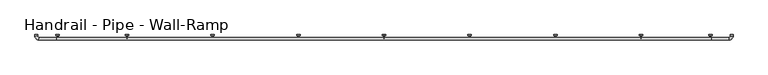
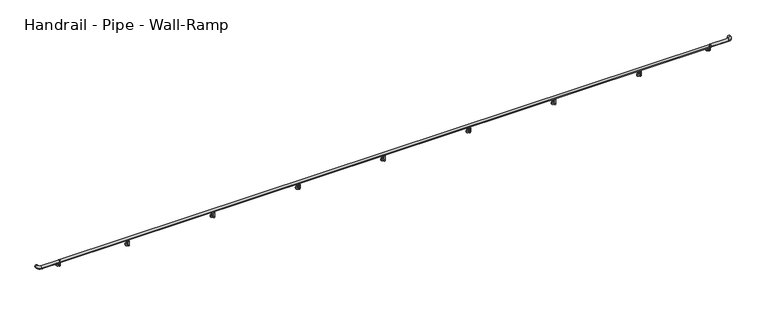
"""IFC4 building model written with IfcOpenShell, lengths in millimetres: railing geometry, Handrail - Pipe - Wall-Ramp."""

from ifc_helpers import new_model, si_unit, point, frame, frame_2d, origin, place, context, project, spatial, circle_curve, ellipse_curve, trimmed, segment, composite_curve, outline, extrude, source, transform, mapped, element, save
from ifc_brep_helpers import plane_surface, cylinder_surface, revolved_surface, advanced_brep


def handrail_pipe_wall_ramp_020da921(model_context):
    return source(origin(), model_context, "Body", "SolidModel", [
        extrude(outline(composite_curve([segment(trimmed(circle_curve(frame_2d((5007.0738685, 895.35)), 19.05), [point((4988.0238685, 895.35))], [point((5026.1238685, 895.35))], False, "CARTESIAN"), True, "CONTINUOUS"), segment(trimmed(circle_curve(frame_2d((5007.0738685, 895.35)), 19.05), [point((5026.1238685, 895.35))], [point((4988.0238685, 895.35))], False, "CARTESIAN"), True, "CONTINUOUS")], self_intersect=False)), frame((-2498.891568, 0.0, 0.0), z_axis=(1.0, 0.0, 0.0), x_axis=(0.0, 1.0, 0.0)), (0.0, 0.0, 1.0), 9315.45),
        advanced_brep(
        [(-1492.416568, 5007.0738685, 857.25), (-1505.116568, 5007.0738685, 857.25), (-1492.416568, 5007.0738685, 800.1), (-1505.116568, 5007.0738685, 800.1), (-1505.116568, 5026.1238685, 781.05), (-1492.416568, 5026.1238685, 781.05), (-1492.416568, 5054.6988685, 781.05), (-1505.116568, 5054.6988685, 781.05)],
        [
            (0, 1, circle_curve(frame((-1498.766568, 5007.0738685, 857.25), z_axis=(0.0, 0.0, 1.0), x_axis=(-1.0, 0.0, 0.0)), 6.35)),
            (1, 0, circle_curve(frame((-1498.766568, 5007.0738685, 857.25), z_axis=(0.0, 0.0, 1.0), x_axis=(-1.0, 0.0, 0.0)), 6.35)),
            (0, 2),
            (2, 3, circle_curve(frame((-1498.766568, 5007.0738685, 800.1), z_axis=(0.0, 0.0, 1.0), x_axis=(-1.0, 0.0, 0.0)), 6.35)),
            (3, 1),
            (3, 2, circle_curve(frame((-1498.766568, 5007.0738685, 800.1), z_axis=(0.0, 0.0, 1.0), x_axis=(-1.0, 0.0, 0.0)), 6.35)),
            (4, 3, circle_curve(frame((-1505.116568, 5026.1238685, 800.1), z_axis=(-1.0, 0.0, 0.0), x_axis=(0.0, -1.0, 0.0)), 19.05)),
            (2, 5, circle_curve(frame((-1492.416568, 5026.1238685, 800.1), z_axis=(1.0, 0.0, 0.0), x_axis=(0.0, -1.0, 0.0)), 19.05)),
            (5, 4, circle_curve(frame((-1498.766568, 5026.1238685, 781.05), z_axis=(0.0, -1.0, 0.0), x_axis=(-1.0, 0.0, 0.0)), 6.35)),
            (4, 5, circle_curve(frame((-1498.766568, 5026.1238685, 781.05), z_axis=(0.0, -1.0, 0.0), x_axis=(-1.0, 0.0, 0.0)), 6.35)),
            (6, 7, circle_curve(frame((-1498.766568, 5054.6988685, 781.05), z_axis=(0.0, 1.0, 0.0), x_axis=(-1.0, 0.0, 0.0)), 6.35)),
            (7, 6, circle_curve(frame((-1498.766568, 5054.6988685, 781.05), z_axis=(0.0, 1.0, 0.0), x_axis=(-1.0, 0.0, 0.0)), 6.35)),
            (5, 6),
            (7, 4),
        ],
        [
            plane_surface(frame((-1505.116568, 5007.0738685, 857.25), z_axis=(0.0, 0.0, 1.0), x_axis=(0.0, 1.0, 0.0))),
            cylinder_surface(frame((-1498.766568, 5007.0738685, 857.25), z_axis=(0.0, 0.0, 1.0), x_axis=(-1.0, 0.0, 0.0)), 6.35),
            revolved_surface(trimmed(ellipse_curve(frame((-1498.766568, 5007.0738685, 800.1), z_axis=(0.0, 0.0, 1.0), x_axis=(-1.0, 0.0, 0.0)), 6.35, 6.35), [point((-1492.416568, 5007.0738685, 800.1))], [point((-1505.116568, 5007.0738685, 800.1))], True, "CARTESIAN"), (-1498.766568, 5026.1238685, 800.1), (1.0, 0.0, 0.0)),
            revolved_surface(trimmed(ellipse_curve(frame((-1498.766568, 5007.0738685, 800.1), z_axis=(0.0, 0.0, 1.0), x_axis=(-1.0, 0.0, 0.0)), 6.35, 6.35), [point((-1505.116568, 5007.0738685, 800.1))], [point((-1492.416568, 5007.0738685, 800.1))], True, "CARTESIAN"), (-1498.766568, 5026.1238685, 800.1), (1.0, 0.0, 0.0)),
            plane_surface(frame((-1498.766568, 5054.6988685, 774.7), z_axis=(0.0, 1.0, 0.0), x_axis=(-1.0, 0.0, 0.0))),
            cylinder_surface(frame((-1498.766568, 5026.1238685, 781.05), z_axis=(0.0, -1.0, 0.0), x_axis=(-1.0, 0.0, 0.0)), 6.35),
        ],
        [
            (0, [[1, 2]]),
            (1, [[-1, 3, 4, 5]]),
            (1, [[-2, -5, 6, -3]]),
            (2, [[7, -4, 8, 9]]),
            (3, [[-8, -6, -7, 10]]),
            (4, [[11, 12]]),
            (5, [[-9, 13, -12, 14]]),
            (5, [[-10, -14, -11, -13]]),
        ],
    ),
        extrude(outline(composite_curve([segment(trimmed(circle_curve(frame_2d((781.05, -1498.766568)), 25.4), [point((781.05, -1524.166568))], [point((781.05, -1473.366568))], False, "CARTESIAN"), True, "CONTINUOUS"), segment(trimmed(circle_curve(frame_2d((781.05, -1498.766568)), 25.4), [point((781.05, -1473.366568))], [point((781.05, -1524.166568))], False, "CARTESIAN"), True, "CONTINUOUS")], self_intersect=False)), frame((0.0, 5054.6988685, 0.0), z_axis=(0.0, 1.0, 0.0), x_axis=(0.0, 0.0, 1.0)), (0.0, 0.0, 1.0), 9.525),
        advanced_brep(
        [(-273.216568, 5007.0738685, 857.25), (-285.916568, 5007.0738685, 857.25), (-273.216568, 5007.0738685, 800.1), (-285.916568, 5007.0738685, 800.1), (-285.916568, 5026.1238685, 781.05), (-273.216568, 5026.1238685, 781.05), (-273.216568, 5054.6988685, 781.05), (-285.916568, 5054.6988685, 781.05)],
        [
            (0, 1, circle_curve(frame((-279.566568, 5007.0738685, 857.25), z_axis=(0.0, 0.0, 1.0), x_axis=(-1.0, 0.0, 0.0)), 6.35)),
            (1, 0, circle_curve(frame((-279.566568, 5007.0738685, 857.25), z_axis=(0.0, 0.0, 1.0), x_axis=(-1.0, 0.0, 0.0)), 6.35)),
            (0, 2),
            (2, 3, circle_curve(frame((-279.566568, 5007.0738685, 800.1), z_axis=(0.0, 0.0, 1.0), x_axis=(-1.0, 0.0, 0.0)), 6.35)),
            (3, 1),
            (3, 2, circle_curve(frame((-279.566568, 5007.0738685, 800.1), z_axis=(0.0, 0.0, 1.0), x_axis=(-1.0, 0.0, 0.0)), 6.35)),
            (4, 3, circle_curve(frame((-285.916568, 5026.1238685, 800.1), z_axis=(-1.0, 0.0, 0.0), x_axis=(0.0, -1.0, 0.0)), 19.05)),
            (2, 5, circle_curve(frame((-273.216568, 5026.1238685, 800.1), z_axis=(1.0, 0.0, 0.0), x_axis=(0.0, -1.0, 0.0)), 19.05)),
            (5, 4, circle_curve(frame((-279.566568, 5026.1238685, 781.05), z_axis=(0.0, -1.0, 0.0), x_axis=(-1.0, 0.0, 0.0)), 6.35)),
            (4, 5, circle_curve(frame((-279.566568, 5026.1238685, 781.05), z_axis=(0.0, -1.0, 0.0), x_axis=(-1.0, 0.0, 0.0)), 6.35)),
            (6, 7, circle_curve(frame((-279.566568, 5054.6988685, 781.05), z_axis=(0.0, 1.0, 0.0), x_axis=(-1.0, 0.0, 0.0)), 6.35)),
            (7, 6, circle_curve(frame((-279.566568, 5054.6988685, 781.05), z_axis=(0.0, 1.0, 0.0), x_axis=(-1.0, 0.0, 0.0)), 6.35)),
            (5, 6),
            (7, 4),
        ],
        [
            plane_surface(frame((-285.916568, 5007.0738685, 857.25), z_axis=(0.0, 0.0, 1.0), x_axis=(0.0, 1.0, 0.0))),
            cylinder_surface(frame((-279.566568, 5007.0738685, 857.25), z_axis=(0.0, 0.0, 1.0), x_axis=(-1.0, 0.0, 0.0)), 6.35),
            revolved_surface(trimmed(ellipse_curve(frame((-279.566568, 5007.0738685, 800.1), z_axis=(0.0, 0.0, 1.0), x_axis=(-1.0, 0.0, 0.0)), 6.35, 6.35), [point((-273.216568, 5007.0738685, 800.1))], [point((-285.916568, 5007.0738685, 800.1))], True, "CARTESIAN"), (-279.566568, 5026.1238685, 800.1), (1.0, 0.0, 0.0)),
            revolved_surface(trimmed(ellipse_curve(frame((-279.566568, 5007.0738685, 800.1), z_axis=(0.0, 0.0, 1.0), x_axis=(-1.0, 0.0, 0.0)), 6.35, 6.35), [point((-285.916568, 5007.0738685, 800.1))], [point((-273.216568, 5007.0738685, 800.1))], True, "CARTESIAN"), (-279.566568, 5026.1238685, 800.1), (1.0, 0.0, 0.0)),
            plane_surface(frame((-279.566568, 5054.6988685, 774.7), z_axis=(0.0, 1.0, 0.0), x_axis=(-1.0, 0.0, 0.0))),
            cylinder_surface(frame((-279.566568, 5026.1238685, 781.05), z_axis=(0.0, -1.0, 0.0), x_axis=(-1.0, 0.0, 0.0)), 6.35),
        ],
        [
            (0, [[1, 2]]),
            (1, [[-1, 3, 4, 5]]),
            (1, [[-2, -5, 6, -3]]),
            (2, [[7, -4, 8, 9]]),
            (3, [[-8, -6, -7, 10]]),
            (4, [[11, 12]]),
            (5, [[-9, 13, -12, 14]]),
            (5, [[-10, -14, -11, -13]]),
        ],
    ),
        extrude(outline(composite_curve([segment(trimmed(circle_curve(frame_2d((781.05, -279.566568)), 25.4), [point((781.05, -304.966568))], [point((781.05, -254.166568))], False, "CARTESIAN"), True, "CONTINUOUS"), segment(trimmed(circle_curve(frame_2d((781.05, -279.566568)), 25.4), [point((781.05, -254.166568))], [point((781.05, -304.966568))], False, "CARTESIAN"), True, "CONTINUOUS")], self_intersect=False)), frame((0.0, 5054.6988685, 0.0), z_axis=(0.0, 1.0, 0.0), x_axis=(0.0, 0.0, 1.0)), (0.0, 0.0, 1.0), 9.525),
        advanced_brep(
        [(945.983432, 5007.0738685, 857.25), (933.283432, 5007.0738685, 857.25), (945.983432, 5007.0738685, 800.1), (933.283432, 5007.0738685, 800.1), (933.283432, 5026.1238685, 781.05), (945.983432, 5026.1238685, 781.05), (945.983432, 5054.6988685, 781.05), (933.283432, 5054.6988685, 781.05)],
        [
            (0, 1, circle_curve(frame((939.633432, 5007.0738685, 857.25), z_axis=(0.0, 0.0, 1.0), x_axis=(-1.0, 0.0, 0.0)), 6.35)),
            (1, 0, circle_curve(frame((939.633432, 5007.0738685, 857.25), z_axis=(0.0, 0.0, 1.0), x_axis=(-1.0, 0.0, 0.0)), 6.35)),
            (0, 2),
            (2, 3, circle_curve(frame((939.633432, 5007.0738685, 800.1), z_axis=(0.0, 0.0, 1.0), x_axis=(-1.0, 0.0, 0.0)), 6.35)),
            (3, 1),
            (3, 2, circle_curve(frame((939.633432, 5007.0738685, 800.1), z_axis=(0.0, 0.0, 1.0), x_axis=(-1.0, 0.0, 0.0)), 6.35)),
            (4, 3, circle_curve(frame((933.283432, 5026.1238685, 800.1), z_axis=(-1.0, 0.0, 0.0), x_axis=(0.0, -1.0, 0.0)), 19.05)),
            (2, 5, circle_curve(frame((945.983432, 5026.1238685, 800.1), z_axis=(1.0, 0.0, 0.0), x_axis=(0.0, -1.0, 0.0)), 19.05)),
            (5, 4, circle_curve(frame((939.633432, 5026.1238685, 781.05), z_axis=(0.0, -1.0, 0.0), x_axis=(-1.0, 0.0, 0.0)), 6.35)),
            (4, 5, circle_curve(frame((939.633432, 5026.1238685, 781.05), z_axis=(0.0, -1.0, 0.0), x_axis=(-1.0, 0.0, 0.0)), 6.35)),
            (6, 7, circle_curve(frame((939.633432, 5054.6988685, 781.05), z_axis=(0.0, 1.0, 0.0), x_axis=(-1.0, 0.0, 0.0)), 6.35)),
            (7, 6, circle_curve(frame((939.633432, 5054.6988685, 781.05), z_axis=(0.0, 1.0, 0.0), x_axis=(-1.0, 0.0, 0.0)), 6.35)),
            (5, 6),
            (7, 4),
        ],
        [
            plane_surface(frame((933.283432, 5007.0738685, 857.25), z_axis=(0.0, 0.0, 1.0), x_axis=(0.0, 1.0, 0.0))),
            cylinder_surface(frame((939.633432, 5007.0738685, 857.25), z_axis=(0.0, 0.0, 1.0), x_axis=(-1.0, 0.0, 0.0)), 6.35),
            revolved_surface(trimmed(ellipse_curve(frame((939.633432, 5007.0738685, 800.1), z_axis=(0.0, 0.0, 1.0), x_axis=(-1.0, 0.0, 0.0)), 6.35, 6.35), [point((945.983432, 5007.0738685, 800.1))], [point((933.283432, 5007.0738685, 800.1))], True, "CARTESIAN"), (939.633432, 5026.1238685, 800.1), (1.0, 0.0, 0.0)),
            revolved_surface(trimmed(ellipse_curve(frame((939.633432, 5007.0738685, 800.1), z_axis=(0.0, 0.0, 1.0), x_axis=(-1.0, 0.0, 0.0)), 6.35, 6.35), [point((933.283432, 5007.0738685, 800.1))], [point((945.983432, 5007.0738685, 800.1))], True, "CARTESIAN"), (939.633432, 5026.1238685, 800.1), (1.0, 0.0, 0.0)),
            plane_surface(frame((939.633432, 5054.6988685, 774.7), z_axis=(0.0, 1.0, 0.0), x_axis=(-1.0, 0.0, 0.0))),
            cylinder_surface(frame((939.633432, 5026.1238685, 781.05), z_axis=(0.0, -1.0, 0.0), x_axis=(-1.0, 0.0, 0.0)), 6.35),
        ],
        [
            (0, [[1, 2]]),
            (1, [[-1, 3, 4, 5]]),
            (1, [[-2, -5, 6, -3]]),
            (2, [[7, -4, 8, 9]]),
            (3, [[-8, -6, -7, 10]]),
            (4, [[11, 12]]),
            (5, [[-9, 13, -12, 14]]),
            (5, [[-10, -14, -11, -13]]),
        ],
    ),
        extrude(outline(composite_curve([segment(trimmed(circle_curve(frame_2d((781.05, 939.633432)), 25.4), [point((781.05, 914.233432))], [point((781.05, 965.033432))], False, "CARTESIAN"), True, "CONTINUOUS"), segment(trimmed(circle_curve(frame_2d((781.05, 939.633432)), 25.4), [point((781.05, 965.033432))], [point((781.05, 914.233432))], False, "CARTESIAN"), True, "CONTINUOUS")], self_intersect=False)), frame((0.0, 5054.6988685, 0.0), z_axis=(0.0, 1.0, 0.0), x_axis=(0.0, 0.0, 1.0)), (0.0, 0.0, 1.0), 9.525),
        advanced_brep(
        [(2165.183432, 5007.0738685, 857.25), (2152.483432, 5007.0738685, 857.25), (2165.183432, 5007.0738685, 800.1), (2152.483432, 5007.0738685, 800.1), (2152.483432, 5026.1238685, 781.05), (2165.183432, 5026.1238685, 781.05), (2165.183432, 5054.6988685, 781.05), (2152.483432, 5054.6988685, 781.05)],
        [
            (0, 1, circle_curve(frame((2158.833432, 5007.0738685, 857.25), z_axis=(0.0, 0.0, 1.0), x_axis=(-1.0, 0.0, 0.0)), 6.35)),
            (1, 0, circle_curve(frame((2158.833432, 5007.0738685, 857.25), z_axis=(0.0, 0.0, 1.0), x_axis=(-1.0, 0.0, 0.0)), 6.35)),
            (0, 2),
            (2, 3, circle_curve(frame((2158.833432, 5007.0738685, 800.1), z_axis=(0.0, 0.0, 1.0), x_axis=(-1.0, 0.0, 0.0)), 6.35)),
            (3, 1),
            (3, 2, circle_curve(frame((2158.833432, 5007.0738685, 800.1), z_axis=(0.0, 0.0, 1.0), x_axis=(-1.0, 0.0, 0.0)), 6.35)),
            (4, 3, circle_curve(frame((2152.483432, 5026.1238685, 800.1), z_axis=(-1.0, 0.0, 0.0), x_axis=(0.0, -1.0, 0.0)), 19.05)),
            (2, 5, circle_curve(frame((2165.183432, 5026.1238685, 800.1), z_axis=(1.0, 0.0, 0.0), x_axis=(0.0, -1.0, 0.0)), 19.05)),
            (5, 4, circle_curve(frame((2158.833432, 5026.1238685, 781.05), z_axis=(0.0, -1.0, 0.0), x_axis=(-1.0, 0.0, 0.0)), 6.35)),
            (4, 5, circle_curve(frame((2158.833432, 5026.1238685, 781.05), z_axis=(0.0, -1.0, 0.0), x_axis=(-1.0, 0.0, 0.0)), 6.35)),
            (6, 7, circle_curve(frame((2158.833432, 5054.6988685, 781.05), z_axis=(0.0, 1.0, 0.0), x_axis=(-1.0, 0.0, 0.0)), 6.35)),
            (7, 6, circle_curve(frame((2158.833432, 5054.6988685, 781.05), z_axis=(0.0, 1.0, 0.0), x_axis=(-1.0, 0.0, 0.0)), 6.35)),
            (5, 6),
            (7, 4),
        ],
        [
            plane_surface(frame((2152.483432, 5007.0738685, 857.25), z_axis=(0.0, 0.0, 1.0), x_axis=(0.0, 1.0, 0.0))),
            cylinder_surface(frame((2158.833432, 5007.0738685, 857.25), z_axis=(0.0, 0.0, 1.0), x_axis=(-1.0, 0.0, 0.0)), 6.35),
            revolved_surface(trimmed(ellipse_curve(frame((2158.833432, 5007.0738685, 800.1), z_axis=(0.0, 0.0, 1.0), x_axis=(-1.0, 0.0, 0.0)), 6.35, 6.35), [point((2165.183432, 5007.0738685, 800.1))], [point((2152.483432, 5007.0738685, 800.1))], True, "CARTESIAN"), (2158.833432, 5026.1238685, 800.1), (1.0, 0.0, 0.0)),
            revolved_surface(trimmed(ellipse_curve(frame((2158.833432, 5007.0738685, 800.1), z_axis=(0.0, 0.0, 1.0), x_axis=(-1.0, 0.0, 0.0)), 6.35, 6.35), [point((2152.483432, 5007.0738685, 800.1))], [point((2165.183432, 5007.0738685, 800.1))], True, "CARTESIAN"), (2158.833432, 5026.1238685, 800.1), (1.0, 0.0, 0.0)),
            plane_surface(frame((2158.833432, 5054.6988685, 774.7), z_axis=(0.0, 1.0, 0.0), x_axis=(-1.0, 0.0, 0.0))),
            cylinder_surface(frame((2158.833432, 5026.1238685, 781.05), z_axis=(0.0, -1.0, 0.0), x_axis=(-1.0, 0.0, 0.0)), 6.35),
        ],
        [
            (0, [[1, 2]]),
            (1, [[-1, 3, 4, 5]]),
            (1, [[-2, -5, 6, -3]]),
            (2, [[7, -4, 8, 9]]),
            (3, [[-8, -6, -7, 10]]),
            (4, [[11, 12]]),
            (5, [[-9, 13, -12, 14]]),
            (5, [[-10, -14, -11, -13]]),
        ],
    ),
        extrude(outline(composite_curve([segment(trimmed(circle_curve(frame_2d((781.05, 2158.833432)), 25.4), [point((781.05, 2133.433432))], [point((781.05, 2184.233432))], False, "CARTESIAN"), True, "CONTINUOUS"), segment(trimmed(circle_curve(frame_2d((781.05, 2158.833432)), 25.4), [point((781.05, 2184.233432))], [point((781.05, 2133.433432))], False, "CARTESIAN"), True, "CONTINUOUS")], self_intersect=False)), frame((0.0, 5054.6988685, 0.0), z_axis=(0.0, 1.0, 0.0), x_axis=(0.0, 0.0, 1.0)), (0.0, 0.0, 1.0), 9.525),
        advanced_brep(
        [(3384.383432, 5007.0738685, 857.25), (3371.683432, 5007.0738685, 857.25), (3384.383432, 5007.0738685, 800.1), (3371.683432, 5007.0738685, 800.1), (3371.683432, 5026.1238685, 781.05), (3384.383432, 5026.1238685, 781.05), (3384.383432, 5054.6988685, 781.05), (3371.683432, 5054.6988685, 781.05)],
        [
            (0, 1, circle_curve(frame((3378.033432, 5007.0738685, 857.25), z_axis=(0.0, 0.0, 1.0), x_axis=(-1.0, 0.0, 0.0)), 6.35)),
            (1, 0, circle_curve(frame((3378.033432, 5007.0738685, 857.25), z_axis=(0.0, 0.0, 1.0), x_axis=(-1.0, 0.0, 0.0)), 6.35)),
            (0, 2),
            (2, 3, circle_curve(frame((3378.033432, 5007.0738685, 800.1), z_axis=(0.0, 0.0, 1.0), x_axis=(-1.0, 0.0, 0.0)), 6.35)),
            (3, 1),
            (3, 2, circle_curve(frame((3378.033432, 5007.0738685, 800.1), z_axis=(0.0, 0.0, 1.0), x_axis=(-1.0, 0.0, 0.0)), 6.35)),
            (4, 3, circle_curve(frame((3371.683432, 5026.1238685, 800.1), z_axis=(-1.0, 0.0, 0.0), x_axis=(0.0, -1.0, 0.0)), 19.05)),
            (2, 5, circle_curve(frame((3384.383432, 5026.1238685, 800.1), z_axis=(1.0, 0.0, 0.0), x_axis=(0.0, -1.0, 0.0)), 19.05)),
            (5, 4, circle_curve(frame((3378.033432, 5026.1238685, 781.05), z_axis=(0.0, -1.0, 0.0), x_axis=(-1.0, 0.0, 0.0)), 6.35)),
            (4, 5, circle_curve(frame((3378.033432, 5026.1238685, 781.05), z_axis=(0.0, -1.0, 0.0), x_axis=(-1.0, 0.0, 0.0)), 6.35)),
            (6, 7, circle_curve(frame((3378.033432, 5054.6988685, 781.05), z_axis=(0.0, 1.0, 0.0), x_axis=(-1.0, 0.0, 0.0)), 6.35)),
            (7, 6, circle_curve(frame((3378.033432, 5054.6988685, 781.05), z_axis=(0.0, 1.0, 0.0), x_axis=(-1.0, 0.0, 0.0)), 6.35)),
            (5, 6),
            (7, 4),
        ],
        [
            plane_surface(frame((3371.683432, 5007.0738685, 857.25), z_axis=(0.0, 0.0, 1.0), x_axis=(0.0, 1.0, 0.0))),
            cylinder_surface(frame((3378.033432, 5007.0738685, 857.25), z_axis=(0.0, 0.0, 1.0), x_axis=(-1.0, 0.0, 0.0)), 6.35),
            revolved_surface(trimmed(ellipse_curve(frame((3378.033432, 5007.0738685, 800.1), z_axis=(0.0, 0.0, 1.0), x_axis=(-1.0, 0.0, 0.0)), 6.35, 6.35), [point((3384.383432, 5007.0738685, 800.1))], [point((3371.683432, 5007.0738685, 800.1))], True, "CARTESIAN"), (3378.033432, 5026.1238685, 800.1), (1.0, 0.0, 0.0)),
            revolved_surface(trimmed(ellipse_curve(frame((3378.033432, 5007.0738685, 800.1), z_axis=(0.0, 0.0, 1.0), x_axis=(-1.0, 0.0, 0.0)), 6.35, 6.35), [point((3371.683432, 5007.0738685, 800.1))], [point((3384.383432, 5007.0738685, 800.1))], True, "CARTESIAN"), (3378.033432, 5026.1238685, 800.1), (1.0, 0.0, 0.0)),
            plane_surface(frame((3378.033432, 5054.6988685, 774.7), z_axis=(0.0, 1.0, 0.0), x_axis=(-1.0, 0.0, 0.0))),
            cylinder_surface(frame((3378.033432, 5026.1238685, 781.05), z_axis=(0.0, -1.0, 0.0), x_axis=(-1.0, 0.0, 0.0)), 6.35),
        ],
        [
            (0, [[1, 2]]),
            (1, [[-1, 3, 4, 5]]),
            (1, [[-2, -5, 6, -3]]),
            (2, [[7, -4, 8, 9]]),
            (3, [[-8, -6, -7, 10]]),
            (4, [[11, 12]]),
            (5, [[-9, 13, -12, 14]]),
            (5, [[-10, -14, -11, -13]]),
        ],
    ),
        extrude(outline(composite_curve([segment(trimmed(circle_curve(frame_2d((781.05, 3378.033432)), 25.4), [point((781.05, 3352.633432))], [point((781.05, 3403.433432))], False, "CARTESIAN"), True, "CONTINUOUS"), segment(trimmed(circle_curve(frame_2d((781.05, 3378.033432)), 25.4), [point((781.05, 3403.433432))], [point((781.05, 3352.633432))], False, "CARTESIAN"), True, "CONTINUOUS")], self_intersect=False)), frame((0.0, 5054.6988685, 0.0), z_axis=(0.0, 1.0, 0.0), x_axis=(0.0, 0.0, 1.0)), (0.0, 0.0, 1.0), 9.525),
        advanced_brep(
        [(4603.583432, 5007.0738685, 857.25), (4590.883432, 5007.0738685, 857.25), (4603.583432, 5007.0738685, 800.1), (4590.883432, 5007.0738685, 800.1), (4590.883432, 5026.1238685, 781.05), (4603.583432, 5026.1238685, 781.05), (4603.583432, 5054.6988685, 781.05), (4590.883432, 5054.6988685, 781.05)],
        [
            (0, 1, circle_curve(frame((4597.233432, 5007.0738685, 857.25), z_axis=(0.0, 0.0, 1.0), x_axis=(-1.0, 0.0, 0.0)), 6.35)),
            (1, 0, circle_curve(frame((4597.233432, 5007.0738685, 857.25), z_axis=(0.0, 0.0, 1.0), x_axis=(-1.0, 0.0, 0.0)), 6.35)),
            (0, 2),
            (2, 3, circle_curve(frame((4597.233432, 5007.0738685, 800.1), z_axis=(0.0, 0.0, 1.0), x_axis=(-1.0, 0.0, 0.0)), 6.35)),
            (3, 1),
            (3, 2, circle_curve(frame((4597.233432, 5007.0738685, 800.1), z_axis=(0.0, 0.0, 1.0), x_axis=(-1.0, 0.0, 0.0)), 6.35)),
            (4, 3, circle_curve(frame((4590.883432, 5026.1238685, 800.1), z_axis=(-1.0, 0.0, 0.0), x_axis=(0.0, -1.0, 0.0)), 19.05)),
            (2, 5, circle_curve(frame((4603.583432, 5026.1238685, 800.1), z_axis=(1.0, 0.0, 0.0), x_axis=(0.0, -1.0, 0.0)), 19.05)),
            (5, 4, circle_curve(frame((4597.233432, 5026.1238685, 781.05), z_axis=(0.0, -1.0, 0.0), x_axis=(-1.0, 0.0, 0.0)), 6.35)),
            (4, 5, circle_curve(frame((4597.233432, 5026.1238685, 781.05), z_axis=(0.0, -1.0, 0.0), x_axis=(-1.0, 0.0, 0.0)), 6.35)),
            (6, 7, circle_curve(frame((4597.233432, 5054.6988685, 781.05), z_axis=(0.0, 1.0, 0.0), x_axis=(-1.0, 0.0, 0.0)), 6.35)),
            (7, 6, circle_curve(frame((4597.233432, 5054.6988685, 781.05), z_axis=(0.0, 1.0, 0.0), x_axis=(-1.0, 0.0, 0.0)), 6.35)),
            (5, 6),
            (7, 4),
        ],
        [
            plane_surface(frame((4590.883432, 5007.0738685, 857.25), z_axis=(0.0, 0.0, 1.0), x_axis=(0.0, 1.0, 0.0))),
            cylinder_surface(frame((4597.233432, 5007.0738685, 857.25), z_axis=(0.0, 0.0, 1.0), x_axis=(-1.0, 0.0, 0.0)), 6.35),
            revolved_surface(trimmed(ellipse_curve(frame((4597.233432, 5007.0738685, 800.1), z_axis=(0.0, 0.0, 1.0), x_axis=(-1.0, 0.0, 0.0)), 6.35, 6.35), [point((4603.583432, 5007.0738685, 800.1))], [point((4590.883432, 5007.0738685, 800.1))], True, "CARTESIAN"), (4597.233432, 5026.1238685, 800.1), (1.0, 0.0, 0.0)),
            revolved_surface(trimmed(ellipse_curve(frame((4597.233432, 5007.0738685, 800.1), z_axis=(0.0, 0.0, 1.0), x_axis=(-1.0, 0.0, 0.0)), 6.35, 6.35), [point((4590.883432, 5007.0738685, 800.1))], [point((4603.583432, 5007.0738685, 800.1))], True, "CARTESIAN"), (4597.233432, 5026.1238685, 800.1), (1.0, 0.0, 0.0)),
            plane_surface(frame((4597.233432, 5054.6988685, 774.7), z_axis=(0.0, 1.0, 0.0), x_axis=(-1.0, 0.0, 0.0))),
            cylinder_surface(frame((4597.233432, 5026.1238685, 781.05), z_axis=(0.0, -1.0, 0.0), x_axis=(-1.0, 0.0, 0.0)), 6.35),
        ],
        [
            (0, [[1, 2]]),
            (1, [[-1, 3, 4, 5]]),
            (1, [[-2, -5, 6, -3]]),
            (2, [[7, -4, 8, 9]]),
            (3, [[-8, -6, -7, 10]]),
            (4, [[11, 12]]),
            (5, [[-9, 13, -12, 14]]),
            (5, [[-10, -14, -11, -13]]),
        ],
    ),
        extrude(outline(composite_curve([segment(trimmed(circle_curve(frame_2d((781.05, 4597.233432)), 25.4), [point((781.05, 4571.833432))], [point((781.05, 4622.633432))], False, "CARTESIAN"), True, "CONTINUOUS"), segment(trimmed(circle_curve(frame_2d((781.05, 4597.233432)), 25.4), [point((781.05, 4622.633432))], [point((781.05, 4571.833432))], False, "CARTESIAN"), True, "CONTINUOUS")], self_intersect=False)), frame((0.0, 5054.6988685, 0.0), z_axis=(0.0, 1.0, 0.0), x_axis=(0.0, 0.0, 1.0)), (0.0, 0.0, 1.0), 9.525),
        advanced_brep(
        [(5822.783432, 5007.0738685, 857.25), (5810.083432, 5007.0738685, 857.25), (5822.783432, 5007.0738685, 800.1), (5810.083432, 5007.0738685, 800.1), (5810.083432, 5026.1238685, 781.05), (5822.783432, 5026.1238685, 781.05), (5822.783432, 5054.6988685, 781.05), (5810.083432, 5054.6988685, 781.05)],
        [
            (0, 1, circle_curve(frame((5816.433432, 5007.0738685, 857.25), z_axis=(0.0, 0.0, 1.0), x_axis=(-1.0, 0.0, 0.0)), 6.35)),
            (1, 0, circle_curve(frame((5816.433432, 5007.0738685, 857.25), z_axis=(0.0, 0.0, 1.0), x_axis=(-1.0, 0.0, 0.0)), 6.35)),
            (0, 2),
            (2, 3, circle_curve(frame((5816.433432, 5007.0738685, 800.1), z_axis=(0.0, 0.0, 1.0), x_axis=(-1.0, 0.0, 0.0)), 6.35)),
            (3, 1),
            (3, 2, circle_curve(frame((5816.433432, 5007.0738685, 800.1), z_axis=(0.0, 0.0, 1.0), x_axis=(-1.0, 0.0, 0.0)), 6.35)),
            (4, 3, circle_curve(frame((5810.083432, 5026.1238685, 800.1), z_axis=(-1.0, 0.0, 0.0), x_axis=(0.0, -1.0, 0.0)), 19.05)),
            (2, 5, circle_curve(frame((5822.783432, 5026.1238685, 800.1), z_axis=(1.0, 0.0, 0.0), x_axis=(0.0, -1.0, 0.0)), 19.05)),
            (5, 4, circle_curve(frame((5816.433432, 5026.1238685, 781.05), z_axis=(0.0, -1.0, 0.0), x_axis=(-1.0, 0.0, 0.0)), 6.35)),
            (4, 5, circle_curve(frame((5816.433432, 5026.1238685, 781.05), z_axis=(0.0, -1.0, 0.0), x_axis=(-1.0, 0.0, 0.0)), 6.35)),
            (6, 7, circle_curve(frame((5816.433432, 5054.6988685, 781.05), z_axis=(0.0, 1.0, 0.0), x_axis=(-1.0, 0.0, 0.0)), 6.35)),
            (7, 6, circle_curve(frame((5816.433432, 5054.6988685, 781.05), z_axis=(0.0, 1.0, 0.0), x_axis=(-1.0, 0.0, 0.0)), 6.35)),
            (5, 6),
            (7, 4),
        ],
        [
            plane_surface(frame((5810.083432, 5007.0738685, 857.25), z_axis=(0.0, 0.0, 1.0), x_axis=(0.0, 1.0, 0.0))),
            cylinder_surface(frame((5816.433432, 5007.0738685, 857.25), z_axis=(0.0, 0.0, 1.0), x_axis=(-1.0, 0.0, 0.0)), 6.35),
            revolved_surface(trimmed(ellipse_curve(frame((5816.433432, 5007.0738685, 800.1), z_axis=(0.0, 0.0, 1.0), x_axis=(-1.0, 0.0, 0.0)), 6.35, 6.35), [point((5822.783432, 5007.0738685, 800.1))], [point((5810.083432, 5007.0738685, 800.1))], True, "CARTESIAN"), (5816.433432, 5026.1238685, 800.1), (1.0, 0.0, 0.0)),
            revolved_surface(trimmed(ellipse_curve(frame((5816.433432, 5007.0738685, 800.1), z_axis=(0.0, 0.0, 1.0), x_axis=(-1.0, 0.0, 0.0)), 6.35, 6.35), [point((5810.083432, 5007.0738685, 800.1))], [point((5822.783432, 5007.0738685, 800.1))], True, "CARTESIAN"), (5816.433432, 5026.1238685, 800.1), (1.0, 0.0, 0.0)),
            plane_surface(frame((5816.433432, 5054.6988685, 774.7), z_axis=(0.0, 1.0, 0.0), x_axis=(-1.0, 0.0, 0.0))),
            cylinder_surface(frame((5816.433432, 5026.1238685, 781.05), z_axis=(0.0, -1.0, 0.0), x_axis=(-1.0, 0.0, 0.0)), 6.35),
        ],
        [
            (0, [[1, 2]]),
            (1, [[-1, 3, 4, 5]]),
            (1, [[-2, -5, 6, -3]]),
            (2, [[7, -4, 8, 9]]),
            (3, [[-8, -6, -7, 10]]),
            (4, [[11, 12]]),
            (5, [[-9, 13, -12, 14]]),
            (5, [[-10, -14, -11, -13]]),
        ],
    ),
        extrude(outline(composite_curve([segment(trimmed(circle_curve(frame_2d((781.05, 5816.433432)), 25.4), [point((781.05, 5791.033432))], [point((781.05, 5841.833432))], False, "CARTESIAN"), True, "CONTINUOUS"), segment(trimmed(circle_curve(frame_2d((781.05, 5816.433432)), 25.4), [point((781.05, 5841.833432))], [point((781.05, 5791.033432))], False, "CARTESIAN"), True, "CONTINUOUS")], self_intersect=False)), frame((0.0, 5054.6988685, 0.0), z_axis=(0.0, 1.0, 0.0), x_axis=(0.0, 0.0, 1.0)), (0.0, 0.0, 1.0), 9.525),
        advanced_brep(
        [(-2486.191568, 5026.1238685, 895.35), (-2486.191568, 4988.0238685, 895.35), (-2752.891568, 5026.1238685, 895.35), (-2752.891568, 4988.0238685, 895.35), (-2810.041568, 5045.1738685, 895.35), (-2771.941568, 5045.1738685, 895.35), (-2771.941568, 5064.2238685, 895.35), (-2810.041568, 5064.2238685, 895.35)],
        [
            (0, 1, circle_curve(frame((-2486.191568, 5007.0738685, 895.35), z_axis=(1.0, 0.0, 0.0), x_axis=(0.0, -1.0, 0.0)), 19.05)),
            (1, 0, circle_curve(frame((-2486.191568, 5007.0738685, 895.35), z_axis=(1.0, 0.0, 0.0), x_axis=(0.0, -1.0, 0.0)), 19.05)),
            (0, 2),
            (2, 3, circle_curve(frame((-2752.891568, 5007.0738685, 895.35), z_axis=(1.0, 0.0, 0.0), x_axis=(0.0, -1.0, 0.0)), 19.05)),
            (3, 1),
            (3, 2, circle_curve(frame((-2752.891568, 5007.0738685, 895.35), z_axis=(1.0, 0.0, 0.0), x_axis=(0.0, -1.0, 0.0)), 19.05)),
            (4, 3, circle_curve(frame((-2752.891568, 5045.1738685, 895.35), z_axis=(0.0, 0.0, 1.0), x_axis=(0.0, -1.0, 0.0)), 57.15)),
            (2, 5, circle_curve(frame((-2752.891568, 5045.1738685, 895.35), z_axis=(0.0, 0.0, -1.0), x_axis=(0.0, -1.0, 0.0)), 19.05)),
            (5, 4, circle_curve(frame((-2790.991568, 5045.1738685, 895.35), z_axis=(0.0, -1.0, 0.0), x_axis=(-1.0, 0.0, 0.0)), 19.05)),
            (4, 5, circle_curve(frame((-2790.991568, 5045.1738685, 895.35), z_axis=(0.0, -1.0, 0.0), x_axis=(-1.0, 0.0, 0.0)), 19.05)),
            (6, 7, circle_curve(frame((-2790.991568, 5064.2238685, 895.35), z_axis=(0.0, 1.0, 0.0), x_axis=(-1.0, 0.0, 0.0)), 19.05)),
            (7, 6, circle_curve(frame((-2790.991568, 5064.2238685, 895.35), z_axis=(0.0, 1.0, 0.0), x_axis=(-1.0, 0.0, 0.0)), 19.05)),
            (5, 6),
            (7, 4),
        ],
        [
            plane_surface(frame((-2486.191568, 5007.0738685, 895.35), z_axis=(1.0, 0.0, 0.0), x_axis=(0.0, 0.0, 1.0))),
            cylinder_surface(frame((-2486.191568, 5007.0738685, 895.35), z_axis=(1.0, 0.0, 0.0), x_axis=(0.0, -1.0, 0.0)), 19.05),
            revolved_surface(trimmed(ellipse_curve(frame((-2752.891568, 5007.0738685, 895.35), z_axis=(1.0, 0.0, 0.0), x_axis=(0.0, -1.0, 0.0)), 19.05, 19.05), [point((-2752.891568, 5026.1238685, 895.35))], [point((-2752.891568, 4988.0238685, 895.35))], True, "CARTESIAN"), (-2752.891568, 5045.1738685, 895.35), (0.0, 0.0, -1.0)),
            revolved_surface(trimmed(ellipse_curve(frame((-2752.891568, 5007.0738685, 895.35), z_axis=(1.0, 0.0, 0.0), x_axis=(0.0, -1.0, 0.0)), 19.05, 19.05), [point((-2752.891568, 4988.0238685, 895.35))], [point((-2752.891568, 5026.1238685, 895.35))], True, "CARTESIAN"), (-2752.891568, 5045.1738685, 895.35), (0.0, 0.0, -1.0)),
            plane_surface(frame((-2790.991568, 5064.2238685, 895.35), z_axis=(0.0, 1.0, 0.0), x_axis=(0.0, 0.0, 1.0))),
            cylinder_surface(frame((-2790.991568, 5045.1738685, 895.35), z_axis=(0.0, -1.0, 0.0), x_axis=(-1.0, 0.0, 0.0)), 19.05),
        ],
        [
            (0, [[1, 2]]),
            (1, [[-1, 3, 4, 5]]),
            (1, [[-2, -5, 6, -3]]),
            (2, [[7, -4, 8, 9]]),
            (3, [[-8, -6, -7, 10]]),
            (4, [[11, 12]]),
            (5, [[-9, 13, -12, 14]]),
            (5, [[-10, -14, -11, -13]]),
        ],
    ),
        advanced_brep(
        [(-2486.191568, 5054.6988685, 812.8), (-2486.191568, 5054.6988685, 825.5), (-2486.191568, 5026.1238685, 812.8), (-2486.191568, 5026.1238685, 825.5), (-2486.191568, 5013.4238685, 838.2), (-2486.191568, 5000.7238685, 838.2), (-2486.191568, 5000.7238685, 895.35), (-2486.191568, 5013.4238685, 895.35)],
        [
            (0, 1, circle_curve(frame((-2486.191568, 5054.6988685, 819.15), z_axis=(0.0, 1.0, 0.0), x_axis=(0.0, 0.0, 1.0)), 6.35)),
            (1, 0, circle_curve(frame((-2486.191568, 5054.6988685, 819.15), z_axis=(0.0, 1.0, 0.0), x_axis=(0.0, 0.0, 1.0)), 6.35)),
            (0, 2),
            (2, 3, circle_curve(frame((-2486.191568, 5026.1238685, 819.15), z_axis=(0.0, 1.0, 0.0), x_axis=(0.0, 0.0, 1.0)), 6.35)),
            (3, 1),
            (3, 2, circle_curve(frame((-2486.191568, 5026.1238685, 819.15), z_axis=(0.0, 1.0, 0.0), x_axis=(0.0, 0.0, 1.0)), 6.35)),
            (4, 3, circle_curve(frame((-2486.191568, 5026.1238685, 838.2), z_axis=(1.0, 0.0, 0.0), x_axis=(0.0, 0.0, -1.0)), 12.7)),
            (2, 5, circle_curve(frame((-2486.191568, 5026.1238685, 838.2), z_axis=(-1.0, 0.0, 0.0), x_axis=(0.0, 0.0, -1.0)), 25.4)),
            (5, 4, circle_curve(frame((-2486.191568, 5007.0738685, 838.2), z_axis=(0.0, 0.0, -1.0), x_axis=(0.0, 1.0, 0.0)), 6.35)),
            (4, 5, circle_curve(frame((-2486.191568, 5007.0738685, 838.2), z_axis=(0.0, 0.0, -1.0), x_axis=(0.0, 1.0, 0.0)), 6.35)),
            (6, 7, circle_curve(frame((-2486.191568, 5007.0738685, 895.35), z_axis=(0.0, 0.0, 1.0), x_axis=(0.0, 1.0, 0.0)), 6.35)),
            (7, 6, circle_curve(frame((-2486.191568, 5007.0738685, 895.35), z_axis=(0.0, 0.0, 1.0), x_axis=(0.0, 1.0, 0.0)), 6.35)),
            (5, 6),
            (7, 4),
        ],
        [
            plane_surface(frame((-2486.191568, 5054.6988685, 819.15), z_axis=(0.0, 1.0, 0.0), x_axis=(-1.0, 0.0, 0.0))),
            cylinder_surface(frame((-2486.191568, 5054.6988685, 819.15), z_axis=(0.0, 1.0, 0.0), x_axis=(0.0, 0.0, 1.0)), 6.35),
            revolved_surface(trimmed(ellipse_curve(frame((-2486.191568, 5026.1238685, 819.15), z_axis=(0.0, 1.0, 0.0), x_axis=(0.0, 0.0, 1.0)), 6.35, 6.35), [point((-2486.191568, 5026.1238685, 812.8))], [point((-2486.191568, 5026.1238685, 825.5))], True, "CARTESIAN"), (-2486.191568, 5026.1238685, 838.2), (-1.0, 0.0, 0.0)),
            revolved_surface(trimmed(ellipse_curve(frame((-2486.191568, 5026.1238685, 819.15), z_axis=(0.0, 1.0, 0.0), x_axis=(0.0, 0.0, 1.0)), 6.35, 6.35), [point((-2486.191568, 5026.1238685, 825.5))], [point((-2486.191568, 5026.1238685, 812.8))], True, "CARTESIAN"), (-2486.191568, 5026.1238685, 838.2), (-1.0, 0.0, 0.0)),
            plane_surface(frame((-2486.191568, 5007.0738685, 895.35), z_axis=(0.0, 0.0, 1.0), x_axis=(-1.0, 0.0, 0.0))),
            cylinder_surface(frame((-2486.191568, 5007.0738685, 838.2), z_axis=(0.0, 0.0, -1.0), x_axis=(0.0, 1.0, 0.0)), 6.35),
        ],
        [
            (0, [[1, 2]]),
            (1, [[-1, 3, 4, 5]]),
            (1, [[-2, -5, 6, -3]]),
            (2, [[7, -4, 8, 9]]),
            (3, [[-8, -6, -7, 10]]),
            (4, [[11, 12]]),
            (5, [[-9, 13, -12, 14]]),
            (5, [[-10, -14, -11, -13]]),
        ],
    ),
        extrude(outline(composite_curve([segment(trimmed(circle_curve(frame_2d((819.15, -2486.191568)), 25.4), [point((819.15, -2511.591568))], [point((819.15, -2460.791568))], False, "CARTESIAN"), True, "CONTINUOUS"), segment(trimmed(circle_curve(frame_2d((819.15, -2486.191568)), 25.4), [point((819.15, -2460.791568))], [point((819.15, -2511.591568))], False, "CARTESIAN"), True, "CONTINUOUS")], self_intersect=False)), frame((0.0, 5054.6988685, 0.0), z_axis=(0.0, 1.0, 0.0), x_axis=(0.0, 0.0, 1.0)), (0.0, 0.0, 1.0), 9.525),
        advanced_brep(
        [(7089.608432, 5064.2238685, 895.35), (7127.708432, 5064.2238685, 895.35), (7089.608432, 5045.1738685, 895.35), (7127.708432, 5045.1738685, 895.35), (7070.558432, 4988.0238685, 895.35), (7070.558432, 5026.1238685, 895.35), (6803.858432, 5026.1238685, 895.35), (6803.858432, 4988.0238685, 895.35)],
        [
            (0, 1, circle_curve(frame((7108.658432, 5064.2238685, 895.35), z_axis=(0.0, 1.0, 0.0), x_axis=(1.0, 0.0, 0.0)), 19.05)),
            (1, 0, circle_curve(frame((7108.658432, 5064.2238685, 895.35), z_axis=(0.0, 1.0, 0.0), x_axis=(1.0, 0.0, 0.0)), 19.05)),
            (0, 2),
            (2, 3, circle_curve(frame((7108.658432, 5045.1738685, 895.35), z_axis=(0.0, 1.0, 0.0), x_axis=(1.0, 0.0, 0.0)), 19.05)),
            (3, 1),
            (3, 2, circle_curve(frame((7108.658432, 5045.1738685, 895.35), z_axis=(0.0, 1.0, 0.0), x_axis=(1.0, 0.0, 0.0)), 19.05)),
            (4, 3, circle_curve(frame((7070.558432, 5045.1738685, 895.35), z_axis=(0.0, 0.0, 1.0), x_axis=(1.0, 0.0, 0.0)), 57.15)),
            (2, 5, circle_curve(frame((7070.558432, 5045.1738685, 895.35), z_axis=(0.0, 0.0, -1.0), x_axis=(1.0, 0.0, 0.0)), 19.05)),
            (5, 4, circle_curve(frame((7070.558432, 5007.0738685, 895.35), z_axis=(1.0, 0.0, 0.0), x_axis=(0.0, -1.0, 0.0)), 19.05)),
            (4, 5, circle_curve(frame((7070.558432, 5007.0738685, 895.35), z_axis=(1.0, 0.0, 0.0), x_axis=(0.0, -1.0, 0.0)), 19.05)),
            (6, 7, circle_curve(frame((6803.858432, 5007.0738685, 895.35), z_axis=(-1.0, 0.0, 0.0), x_axis=(0.0, -1.0, 0.0)), 19.05)),
            (7, 6, circle_curve(frame((6803.858432, 5007.0738685, 895.35), z_axis=(-1.0, 0.0, 0.0), x_axis=(0.0, -1.0, 0.0)), 19.05)),
            (5, 6),
            (7, 4),
        ],
        [
            plane_surface(frame((7108.658432, 5064.2238685, 895.35), z_axis=(0.0, 1.0, 0.0), x_axis=(0.0, 0.0, 1.0))),
            cylinder_surface(frame((7108.658432, 5064.2238685, 895.35), z_axis=(0.0, 1.0, 0.0), x_axis=(1.0, 0.0, 0.0)), 19.05),
            revolved_surface(trimmed(ellipse_curve(frame((7108.658432, 5045.1738685, 895.35), z_axis=(0.0, 1.0, 0.0), x_axis=(1.0, 0.0, 0.0)), 19.05, 19.05), [point((7089.608432, 5045.1738685, 895.35))], [point((7127.708432, 5045.1738685, 895.35))], True, "CARTESIAN"), (7070.558432, 5045.1738685, 895.35), (0.0, 0.0, -1.0)),
            revolved_surface(trimmed(ellipse_curve(frame((7108.658432, 5045.1738685, 895.35), z_axis=(0.0, 1.0, 0.0), x_axis=(1.0, 0.0, 0.0)), 19.05, 19.05), [point((7127.708432, 5045.1738685, 895.35))], [point((7089.608432, 5045.1738685, 895.35))], True, "CARTESIAN"), (7070.558432, 5045.1738685, 895.35), (0.0, 0.0, -1.0)),
            plane_surface(frame((6803.858432, 5007.0738685, 895.35), z_axis=(-1.0, 0.0, 0.0), x_axis=(0.0, 0.0, 1.0))),
            cylinder_surface(frame((7070.558432, 5007.0738685, 895.35), z_axis=(1.0, 0.0, 0.0), x_axis=(0.0, -1.0, 0.0)), 19.05),
        ],
        [
            (0, [[1, 2]]),
            (1, [[-1, 3, 4, 5]]),
            (1, [[-2, -5, 6, -3]]),
            (2, [[7, -4, 8, 9]]),
            (3, [[-8, -6, -7, 10]]),
            (4, [[11, 12]]),
            (5, [[-9, 13, -12, 14]]),
            (5, [[-10, -14, -11, -13]]),
        ],
    ),
        advanced_brep(
        [(6803.858432, 5054.6988685, 812.8), (6803.858432, 5054.6988685, 825.5), (6803.858432, 5026.1238685, 812.8), (6803.858432, 5026.1238685, 825.5), (6803.858432, 5013.4238685, 838.2), (6803.858432, 5000.7238685, 838.2), (6803.858432, 5000.7238685, 895.35), (6803.858432, 5013.4238685, 895.35)],
        [
            (0, 1, circle_curve(frame((6803.858432, 5054.6988685, 819.15), z_axis=(0.0, 1.0, 0.0), x_axis=(0.0, 0.0, 1.0)), 6.35)),
            (1, 0, circle_curve(frame((6803.858432, 5054.6988685, 819.15), z_axis=(0.0, 1.0, 0.0), x_axis=(0.0, 0.0, 1.0)), 6.35)),
            (0, 2),
            (2, 3, circle_curve(frame((6803.858432, 5026.1238685, 819.15), z_axis=(0.0, 1.0, 0.0), x_axis=(0.0, 0.0, 1.0)), 6.35)),
            (3, 1),
            (3, 2, circle_curve(frame((6803.858432, 5026.1238685, 819.15), z_axis=(0.0, 1.0, 0.0), x_axis=(0.0, 0.0, 1.0)), 6.35)),
            (4, 3, circle_curve(frame((6803.858432, 5026.1238685, 838.2), z_axis=(1.0, 0.0, 0.0), x_axis=(0.0, 0.0, -1.0)), 12.7)),
            (2, 5, circle_curve(frame((6803.858432, 5026.1238685, 838.2), z_axis=(-1.0, 0.0, 0.0), x_axis=(0.0, 0.0, -1.0)), 25.4)),
            (5, 4, circle_curve(frame((6803.858432, 5007.0738685, 838.2), z_axis=(0.0, 0.0, -1.0), x_axis=(0.0, 1.0, 0.0)), 6.35)),
            (4, 5, circle_curve(frame((6803.858432, 5007.0738685, 838.2), z_axis=(0.0, 0.0, -1.0), x_axis=(0.0, 1.0, 0.0)), 6.35)),
            (6, 7, circle_curve(frame((6803.858432, 5007.0738685, 895.35), z_axis=(0.0, 0.0, 1.0), x_axis=(0.0, 1.0, 0.0)), 6.35)),
            (7, 6, circle_curve(frame((6803.858432, 5007.0738685, 895.35), z_axis=(0.0, 0.0, 1.0), x_axis=(0.0, 1.0, 0.0)), 6.35)),
            (5, 6),
            (7, 4),
        ],
        [
            plane_surface(frame((6803.858432, 5054.6988685, 819.15), z_axis=(0.0, 1.0, 0.0), x_axis=(-1.0, 0.0, 0.0))),
            cylinder_surface(frame((6803.858432, 5054.6988685, 819.15), z_axis=(0.0, 1.0, 0.0), x_axis=(0.0, 0.0, 1.0)), 6.35),
            revolved_surface(trimmed(ellipse_curve(frame((6803.858432, 5026.1238685, 819.15), z_axis=(0.0, 1.0, 0.0), x_axis=(0.0, 0.0, 1.0)), 6.35, 6.35), [point((6803.858432, 5026.1238685, 812.8))], [point((6803.858432, 5026.1238685, 825.5))], True, "CARTESIAN"), (6803.858432, 5026.1238685, 838.2), (-1.0, 0.0, 0.0)),
            revolved_surface(trimmed(ellipse_curve(frame((6803.858432, 5026.1238685, 819.15), z_axis=(0.0, 1.0, 0.0), x_axis=(0.0, 0.0, 1.0)), 6.35, 6.35), [point((6803.858432, 5026.1238685, 825.5))], [point((6803.858432, 5026.1238685, 812.8))], True, "CARTESIAN"), (6803.858432, 5026.1238685, 838.2), (-1.0, 0.0, 0.0)),
            plane_surface(frame((6803.858432, 5007.0738685, 895.35), z_axis=(0.0, 0.0, 1.0), x_axis=(-1.0, 0.0, 0.0))),
            cylinder_surface(frame((6803.858432, 5007.0738685, 838.2), z_axis=(0.0, 0.0, -1.0), x_axis=(0.0, 1.0, 0.0)), 6.35),
        ],
        [
            (0, [[1, 2]]),
            (1, [[-1, 3, 4, 5]]),
            (1, [[-2, -5, 6, -3]]),
            (2, [[7, -4, 8, 9]]),
            (3, [[-8, -6, -7, 10]]),
            (4, [[11, 12]]),
            (5, [[-9, 13, -12, 14]]),
            (5, [[-10, -14, -11, -13]]),
        ],
    ),
        extrude(outline(composite_curve([segment(trimmed(circle_curve(frame_2d((819.15, 6803.858432)), 25.4), [point((819.15, 6778.458432))], [point((819.15, 6829.258432))], False, "CARTESIAN"), True, "CONTINUOUS"), segment(trimmed(circle_curve(frame_2d((819.15, 6803.858432)), 25.4), [point((819.15, 6829.258432))], [point((819.15, 6778.458432))], False, "CARTESIAN"), True, "CONTINUOUS")], self_intersect=False)), frame((0.0, 5054.6988685, 0.0), z_axis=(0.0, 1.0, 0.0), x_axis=(0.0, 0.0, 1.0)), (0.0, 0.0, 1.0), 9.525),
    ])


if __name__ == "__main__":
    model = new_model("IFC4")
    model_context = context("Model", 3, world=origin())
    ifc_project = project(units=[si_unit("LENGTHUNIT", "METRE", prefix="MILLI")], contexts=[model_context])
    site = spatial("IfcSite", under=ifc_project)
    building = spatial("IfcBuilding", under=site)
    placement = place(None, origin())
    handrail_pipe_wall_ramp_shape = handrail_pipe_wall_ramp_020da921(model_context)
    element("IfcRailing", 1, ObjectType="Handrail - Pipe - Wall-Ramp", at=placement, inside=building, context=model_context, shape_type="MappedRepresentation", body=[
        mapped(handrail_pipe_wall_ramp_shape, transform((0.0, 0.0, 0.0), x_axis=(1.0, 0.0, 0.0), y_axis=(0.0, 1.0, 0.0), z_axis=(0.0, 0.0, 1.0))),
    ])
    save(model, "model.ifc")

# Revit data of these elements
# Project information
#   Project Issue Date = "Issue Date"
#   Project Status = "Project Status"
#   Client Name = "Owner"
#   Project Address = "Enter address here"
#   Project Name = "Project Name"
#   Project Number = "Project Number"
